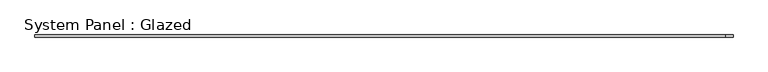
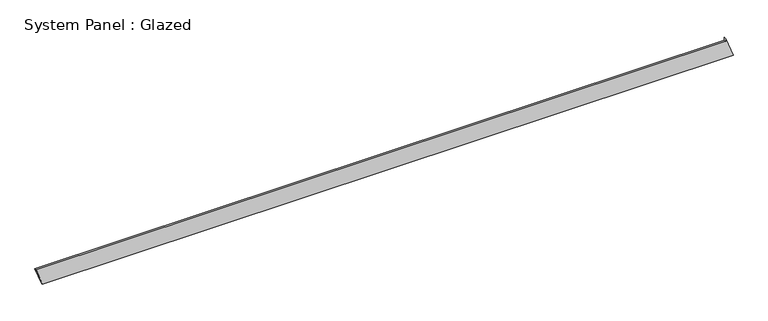
"""IFC4 building model written with IfcOpenShell, lengths in millimetres: plate geometry, System Panel : Glazed."""

import ifcopenshell
import ifcopenshell.guid

model = None  # the IFC model being written
_history = None  # IfcOwnerHistory: only IFC2X3 demands one
_inside = {}  # id of a spatial element -> (the spatial element, [elements in it])
_under = {}  # id of a project, library or spatial element -> (it, [spatial elements below it])
_declared = {}  # id of a project -> (the project, [libraries it declares])
_typed = {}  # id of a type object -> (the type object, [elements of that type])
_made_of = {}  # id of a material, layer set ... -> (it, [elements and type objects made of it])


def new_model(schema):
    """Start an empty IFC model of exactly this schema.

    Asked for "IFC4X3", IfcOpenShell would pick the latest addendum, in which some entities
    have other attributes; the version numbers below select the first issue.
    IFC2X3 requires an IfcOwnerHistory on every rooted entity: one is made here for all.
    """
    global model, _history
    if schema == "IFC4X3":
        model = ifcopenshell.file(schema_version=(4, 3, 0, 0))
    else:
        model = ifcopenshell.file(schema=schema)
    _inside.clear()
    _under.clear()
    _declared.clear()
    _typed.clear()
    _made_of.clear()
    _history = None
    if model.schema == "IFC2X3":
        org = make("IfcOrganization", Name="unknown")
        user = make(
            "IfcPersonAndOrganization",
            ThePerson=make("IfcPerson", FamilyName="unknown"),
            TheOrganization=org,
        )
        app = make(
            "IfcApplication",
            ApplicationDeveloper=org,
            Version="unknown",
            ApplicationFullName="unknown",
            ApplicationIdentifier="unknown",
        )
        _history = make(
            "IfcOwnerHistory",
            OwningUser=user,
            OwningApplication=app,
            ChangeAction="ADDED",
            CreationDate=0,
        )
    return model


def make(cls, **values):
    """One entity of the class cls with the attributes given. An attribute that is None is left unset."""
    return model.create_entity(
        cls, **{name: value for name, value in values.items() if value is not None}
    )


def rooted(cls, **values):
    """An entity with a GlobalId (a new one), such as an element, a storey or a relation."""
    return make(cls, GlobalId=ifcopenshell.guid.new(), OwnerHistory=_history, **values)


def si_unit(unit_type, name, prefix=None):
    """IfcSIUnit, for example si_unit("LENGTHUNIT", "METRE", prefix="MILLI")."""
    return make("IfcSIUnit", UnitType=unit_type, Prefix=prefix, Name=name)


def assignment(units):
    """IfcUnitAssignment: the units of a project."""
    return None if units is None else make("IfcUnitAssignment", Units=units)


def point(xyz):
    """IfcCartesianPoint."""
    return None if xyz is None else make("IfcCartesianPoint", Coordinates=xyz)


def direction(xyz):
    """IfcDirection."""
    return None if xyz is None else make("IfcDirection", DirectionRatios=xyz)


def frame(location, z_axis=None, x_axis=None):
    """IfcAxis2Placement3D, a coordinate frame: its origin and axes. An axis left out is left unset."""
    return make(
        "IfcAxis2Placement3D",
        Location=point(location),
        Axis=direction(z_axis),
        RefDirection=direction(x_axis),
    )


def origin():
    """The frame at (0, 0, 0) with its axes left unset."""
    return frame((0.0, 0.0, 0.0))


def place(relative_to, where):
    """IfcLocalPlacement: puts the frame where relative to a parent placement (None: the world)."""
    return make(
        "IfcLocalPlacement", PlacementRelTo=relative_to, RelativePlacement=where
    )


def context(
    kind, dimensions, precision=None, world=None, true_north=None, identifier=None
):
    """IfcGeometricRepresentationContext, for example the 3D "Model" context."""
    return make(
        "IfcGeometricRepresentationContext",
        ContextIdentifier=identifier,
        ContextType=kind,
        CoordinateSpaceDimension=dimensions,
        Precision=precision,
        WorldCoordinateSystem=world,
        TrueNorth=true_north,
    )


def project(units=None, contexts=None):
    """IfcProject with its units and contexts."""
    return rooted(
        "IfcProject",
        Name="project",
        RepresentationContexts=contexts,
        UnitsInContext=assignment(units),
    )


def spatial(cls, under=None, at=None, **own):
    """A site, building, storey or space (cls), placed at a placement, below another one or the project."""
    s = rooted(cls, ObjectPlacement=at, **own)
    if under is not None:
        _under.setdefault(under.id(), (under, []))[1].append(s)
    return s


def polyline(points):
    """IfcPolyline through the points."""
    return make("IfcPolyline", Points=[point(p) for p in points])


def outline(outer, holes=None, kind="AREA"):
    """IfcArbitraryClosedProfileDef: a profile drawn as a closed curve; with holes, ...WithVoids."""
    if holes is None:
        return make("IfcArbitraryClosedProfileDef", ProfileType=kind, OuterCurve=outer)
    return make(
        "IfcArbitraryProfileDefWithVoids",
        ProfileType=kind,
        OuterCurve=outer,
        InnerCurves=holes,
    )


def extrude(swept, where, along, depth):
    """IfcExtrudedAreaSolid: the profile swept, set in the frame where, extruded along a direction by depth."""
    return make(
        "IfcExtrudedAreaSolid",
        SweptArea=swept,
        Position=where,
        ExtrudedDirection=direction(along),
        Depth=depth,
    )


def shape(context_of_items, identifier, shape_type, items):
    """IfcShapeRepresentation: the items that make up one representation, for example the "Body"."""
    return make(
        "IfcShapeRepresentation",
        ContextOfItems=context_of_items,
        RepresentationIdentifier=identifier,
        RepresentationType=shape_type,
        Items=items,
    )


def source(mapping_origin, context_of_items, identifier, shape_type, items):
    """IfcRepresentationMap: a shape defined once, which mapped items show again and again."""
    return make(
        "IfcRepresentationMap",
        MappingOrigin=mapping_origin,
        MappedRepresentation=shape(context_of_items, identifier, shape_type, items),
    )


def transform(
    local_origin,
    x_axis=None,
    y_axis=None,
    z_axis=None,
    scale=None,
    scale2=None,
    scale3=None,
    uniform=True,
):
    """IfcCartesianTransformationOperator3D, or its non-uniform kind. x_axis, y_axis, z_axis: its Axis1, 2, 3."""
    if uniform:
        return make(
            "IfcCartesianTransformationOperator3D",
            Axis1=direction(x_axis),
            Axis2=direction(y_axis),
            LocalOrigin=point(local_origin),
            Scale=scale,
            Axis3=direction(z_axis),
        )
    return make(
        "IfcCartesianTransformationOperator3DnonUniform",
        Axis1=direction(x_axis),
        Axis2=direction(y_axis),
        LocalOrigin=point(local_origin),
        Scale=scale,
        Axis3=direction(z_axis),
        Scale2=scale2,
        Scale3=scale3,
    )


def mapped(mapping_source, mapping_target):
    """IfcMappedItem: shows the shape of a source again, moved by a transform."""
    return make(
        "IfcMappedItem", MappingSource=mapping_source, MappingTarget=mapping_target
    )


def made_of(thing, what):
    """Note that an element or type object is made of a material, layer set ...; save() writes the relation."""
    if what is not None:
        _made_of.setdefault(what.id(), (what, []))[1].append(thing)
    return thing


def element(
    cls,
    number,
    at=None,
    inside=None,
    cuts=None,
    type_object=None,
    material=None,
    context=None,
    identifier="Body",
    shape_type=None,
    held_by="IfcProductDefinitionShape",
    body=None,
    shapes=None,
    **own,
):
    """One element of the class cls, such as IfcWall. Its Tag is "e" and its number.

    at: its placement. inside: the storey or other place that contains it. cuts: it is an
    opening in that element (IfcRelVoidsElement). A single representation is given by context,
    identifier, shape_type and body (its items); several are given by shapes. held_by: the class
    of the entity that holds the representations. save() writes the other relations.
    """
    e = rooted(cls, Tag="e%d" % number, ObjectPlacement=at, **own)
    if body is not None:
        shapes = [shape(context, identifier, shape_type, body)]
    if shapes is not None:
        e.Representation = make(held_by, Representations=shapes)
    if inside is not None:
        _inside.setdefault(inside.id(), (inside, []))[1].append(e)
    if cuts is not None:
        rooted(
            "IfcRelVoidsElement", RelatingBuildingElement=cuts, RelatedOpeningElement=e
        )
    if type_object is not None:
        _typed.setdefault(type_object.id(), (type_object, []))[1].append(e)
    return made_of(e, material)


def aggregate(whole, parts):
    """IfcRelAggregates: a whole, such as a stair, and the parts it consists of."""
    return rooted("IfcRelAggregates", RelatingObject=whole, RelatedObjects=parts)


def save(model, path):
    """Write the relations noted so far, then the file.

    IfcRelAggregates (storeys below a building ...), IfcRelContainedInSpatialStructure (elements
    in a storey), IfcRelDefinesByType, IfcRelAssociatesMaterial and IfcRelDeclares: one each for
    every whole, place, type object, material and project.
    """
    for whole, parts in _under.values():
        aggregate(whole, parts)
    for where, things in _inside.values():
        rooted(
            "IfcRelContainedInSpatialStructure",
            RelatedElements=things,
            RelatingStructure=where,
        )
    for kind, things in _typed.values():
        rooted("IfcRelDefinesByType", RelatedObjects=things, RelatingType=kind)
    for what, things in _made_of.values():
        rooted("IfcRelAssociatesMaterial", RelatedObjects=things, RelatingMaterial=what)
    for by, libraries in _declared.values():
        rooted("IfcRelDeclares", RelatingContext=by, RelatedDefinitions=libraries)
    model.write(path)


def system_panel_glazed_701bf6f3(model_context):
    return source(origin(), model_context, "Body", "SweptSolid", [
        extrude(outline(polyline([(0.0, -3964.1196538), (0.0, 4035.4320594), (234.126736, 3950.0305658), (198.7713971, 3950.02827), (199.28994, -4035.4320594), (0.0, -3964.1196538)])), frame((0.0, -49.5, 0.0), z_axis=(0.0, 1.0, 0.0), x_axis=(0.0, 0.0, 1.0)), (0.0, 0.0, 1.0), 25.0),
    ])


if __name__ == "__main__":
    model = new_model("IFC4")
    model_context = context("Model", 3, world=origin())
    ifc_project = project(units=[si_unit("LENGTHUNIT", "METRE", prefix="MILLI")], contexts=[model_context])
    site = spatial("IfcSite", under=ifc_project)
    building = spatial("IfcBuilding", under=site)
    placement = place(None, origin())
    system_panel_glazed_shape = system_panel_glazed_701bf6f3(model_context)
    element("IfcPlate", 1, ObjectType="System Panel : Glazed", at=placement, inside=building, context=model_context, shape_type="MappedRepresentation", body=[
        mapped(system_panel_glazed_shape, transform((0.0, 0.0, 0.0), x_axis=(1.0, 0.0, 0.0), y_axis=(0.0, 1.0, 0.0), z_axis=(0.0, 0.0, 1.0))),
    ])
    save(model, "model.ifc")

# Revit data of these elements
# Element 1 (IfcPlate, "System Panel : Glazed")
#   Materials on its faces: "Glass"
# Materials
#   "Glass": class "Glass", colour RGB 218 227 224, transparency 0.85, Description = "Soda Lime Glass", Cost = 0
